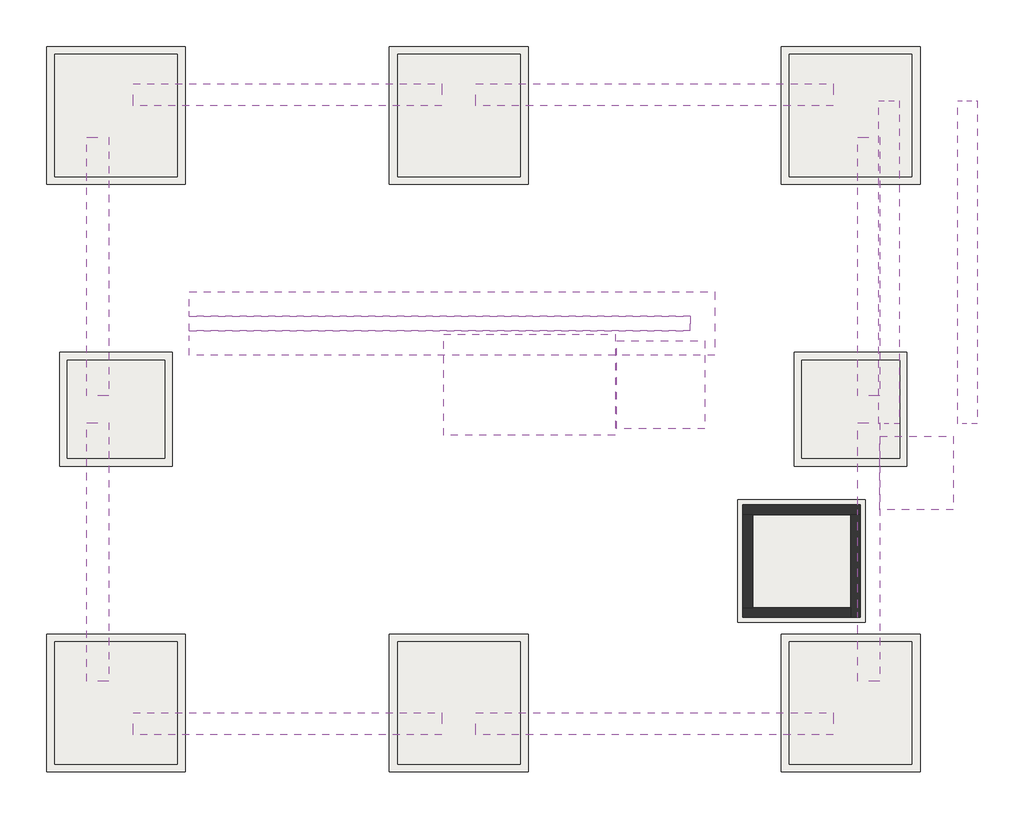
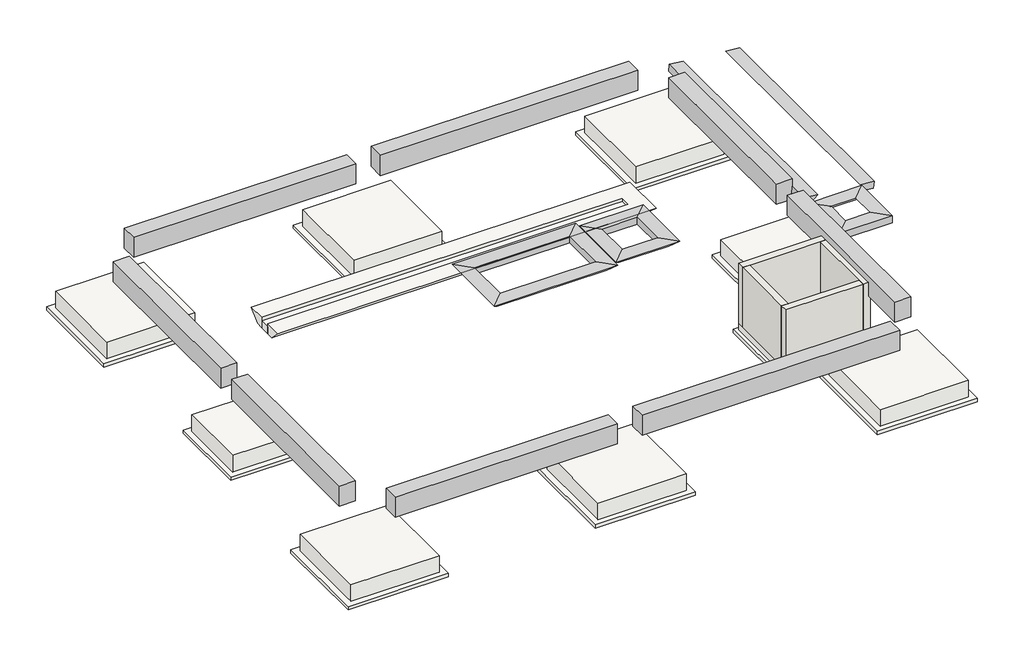
# One storey: 20 slabs, 7 beams, 5 proxies, 4 walls, 1 member.
# Revit data of these elements (continued)
# Type "FT112-Footing-Rectangular : FT112_2500x2500x500" (continued)
#   Foundation Thickness = 500 mm
#   hec_material3 [instance default] = none
#   hec_material2 [instance default] = A03AE056-00001_Bitumen/Bituminous/Asphalt Coating
#   hec_material1 [instance default] = A03AC035-00001_Form Work (3 times in use)_Flat
#   Structural Material [instance default] = A03AC032-00007_Structural Concrete_Type1_25MPa-30Mpa
#   Assembly Code = ""
# Type "MF111_THK.200"
#   Type Comments = ""
#   Layers, outside or top first: 200 mm "A03AC032-00007_Structural Concrete_Type1_25MPa-30Mpa" (function 1); 0 mm "A03AC035-00001_Form Work (3 times in use)_Flat" (function 100); 0 mm "A03AE056-00001_Bitumen/Bituminous/Asphalt Coating" (function 100)
# Type "WA111-UG RC Wall 200mm"
#   Type Comments = ""
#   Layers, outside or top first: 0 mm "A03AE056-00001_Bitumen/Bituminous/Asphalt Coating" (function 100); 200 mm "A03AC032-00007_Structural Concrete_Type1_25MPa-30Mpa" (function 1); 0 mm "A03AC035-00001_Form Work (3 times in use)_Flat" (function 100)
# Elements 1, 2, 3, 4, 5, 6, 7 (IfcBeam, "Concrete-Rectangular-Beam : BM112_450x600_UG")
#   Comments = ""
#   F01) Building Name = "Fire Water Pump Building"
#   F11) Project Building Tag_Type-1 = ""
#   F12) Project Building Tag_Type-2 = ""
#   F13) Project Facility Code = "621"
#   F21) Structural Type = "Steel"
#   F31) Standard Building Code = "E204"
#   F41) Discipline = "Architecture"
#   F51) Plan Start Date-Engineering = "2018-09-14"
#   F52) Plan Finish Date-Engineering = "2019-12-02"
#   F53) Duration = "444"
#   W11) Activity ID = "T3C621AR3610"
#   W12) Activity Name = "Fire Water Pump BLDG - Pedestal/Girder (U/G)"
#   W13) Plan Start Date = "2018-11-20"
#   W14) Plan Finish Date = "2019-02-02"
#   hec_material3 = none
#   hec_material2 = A03AE056-00001_Bitumen/Bituminous/Asphalt Coating
#   hec_material1 = A03AC035-00001_Form Work (3 times in use)_Flat
#   Structural Material = A03AC032-00007_Structural Concrete_Type1_25MPa-30Mpa
#   Phase Created = New Construction
#   Materials on its faces: "A03AC032-00007_Structural Concrete_Type1_25MPa-30Mpa"
# Elements 8, 9, 12 (IfcBuildingElementProxy, "Slab Edge")
#   Phase Created = New Construction
#   Materials on its faces: "Default Floor"
# Element 10 (IfcBuildingElementProxy, "Slab Edge")
#   built-in parameter 1001817 = -0.0996583 (stored number, unit not read)
#   Phase Created = New Construction
#   Materials on its faces: "Default Floor"
# Element 11 (IfcBuildingElementProxy, "Slab Edge")
#   built-in parameter 1001817 = 0.0996583 (stored number, unit not read)
#   Phase Created = New Construction
#   Materials on its faces: "Default Floor"
# Element 13 (IfcMember, "Concrete-Rectangular-Beam : BM112_450x600_UG")
#   Comments = ""
#   F01) Building Name = "Fire Water Pump Building"
#   F11) Project Building Tag_Type-1 = ""
#   F12) Project Building Tag_Type-2 = ""
#   F13) Project Facility Code = "621"
#   F21) Structural Type = "Steel"
#   F31) Standard Building Code = "E204"
#   F41) Discipline = "Architecture"
#   F51) Plan Start Date-Engineering = "2018-09-14"
#   F52) Plan Finish Date-Engineering = "2019-12-02"
#   F53) Duration = "444"
#   W11) Activity ID = "T3C621AR3610"
#   W12) Activity Name = "Fire Water Pump BLDG - Pedestal/Girder (U/G)"
#   W13) Plan Start Date = "2018-11-20"
#   W14) Plan Finish Date = "2019-02-02"
#   hec_material3 = none
#   hec_material2 = A03AE056-00001_Bitumen/Bituminous/Asphalt Coating
#   hec_material1 = A03AC035-00001_Form Work (3 times in use)_Flat
#   Structural Material = A03AC032-00007_Structural Concrete_Type1_25MPa-30Mpa
#   Phase Created = New Construction
#   Materials on its faces: "A03AC032-00007_Structural Concrete_Type1_25MPa-30Mpa"
# Elements 14, 15, 16, 17, 18, 19, 20, 21, 22 (IfcSlab, "SL101_Lean Floor_100")
#   Comments = ""
#   F01) Building Name = "Fire Water Pump Building"
#   F11) Project Building Tag_Type-1 = ""
#   F12) Project Building Tag_Type-2 = ""
#   F13) Project Facility Code = "621"
#   F21) Structural Type = "Steel"
#   F31) Standard Building Code = "E204"
#   F41) Discipline = "Architecture"
#   F51) Plan Start Date-Engineering = "2018-09-14"
#   F52) Plan Finish Date-Engineering = "2019-12-02"
#   F53) Duration = "444"
#   W11) Activity ID = "T3C621AR3110"
#   W12) Activity Name = "Fire Water Pump BLDG - Building Foundation"
#   W13) Plan Start Date = "2018-10-02"
#   W14) Plan Finish Date = "2018-11-24"
#   TMP_Element Name = "SS2"
#   Height Offset From Level = 0 mm
#   built-in parameter 1001954 = 1
#   Phase Created = New Construction
#   Materials on its faces: "A03AC034-00004_Lean Concrete (including Form work)"
# Element 23 (IfcSlab, "Ditch Wall 1 : Ditch Wall 1")
#   Phase Created = New Construction
#   Materials on its faces: "A03AC032-00007_Structural Concrete_Type1_25MPa-30Mpa"
# Element 24 (IfcSlab, "Ditch 2 : Ditch 2")
#   Phase Created = New Construction
#   Materials on its faces: "A03AC032-00007_Structural Concrete_Type1_25MPa-30Mpa"
# Elements 25, 26 (IfcSlab, "FT112-Footing-Rectangular : FT112_2000x2000x500")
#   Comments = ""
#   Mark = "F3"
#   F01) Building Name = "Fire Water Pump Building"
#   F11) Project Building Tag_Type-1 = ""
#   F12) Project Building Tag_Type-2 = ""
#   F13) Project Facility Code = "621"
#   F21) Structural Type = "Steel"
#   F31) Standard Building Code = "E204"
#   F41) Discipline = "Architecture"
#   F51) Plan Start Date-Engineering = "2018-09-14"
#   F52) Plan Finish Date-Engineering = "2019-12-02"
#   F53) Duration = "444"
#   W11) Activity ID = "T3C621AR3110"
#   W12) Activity Name = "Fire Water Pump BLDG - Building Foundation"
#   W13) Plan Start Date = "2018-10-02"
#   W14) Plan Finish Date = "2018-11-24"
#   Structural Material = 콘크리트 - 현장타설 콘크리트
#   Phase Created = New Construction
#   Materials on its faces: "콘크리트 - 현장타설 콘크리트"
# Elements 27, 28, 30, 31 (IfcSlab, "FT112-Footing-Rectangular : FT112_2500x2500x500")
#   Comments = ""
#   Mark = "F2"
#   F01) Building Name = "Fire Water Pump Building"
#   F11) Project Building Tag_Type-1 = ""
#   F12) Project Building Tag_Type-2 = ""
#   F13) Project Facility Code = "621"
#   F21) Structural Type = "Steel"
#   F31) Standard Building Code = "E204"
#   F41) Discipline = "Architecture"
#   F51) Plan Start Date-Engineering = "2018-09-14"
#   F52) Plan Finish Date-Engineering = "2019-12-02"
#   F53) Duration = "444"
#   W11) Activity ID = "T3C621AR3110"
#   W12) Activity Name = "Fire Water Pump BLDG - Building Foundation"
#   W13) Plan Start Date = "2018-10-02"
#   W14) Plan Finish Date = "2018-11-24"
#   Structural Material = 콘크리트 - 현장타설 콘크리트
#   Phase Created = New Construction
#   Materials on its faces: "콘크리트 - 현장타설 콘크리트"
# Elements 29, 32 (IfcSlab, "FT112-Footing-Rectangular : FT112_2500x2500x500")
#   Comments = ""
#   Mark = "F1"
#   F01) Building Name = "Fire Water Pump Building"
#   F11) Project Building Tag_Type-1 = ""
#   F12) Project Building Tag_Type-2 = ""
#   F13) Project Facility Code = "621"
#   F21) Structural Type = "Steel"
#   F31) Standard Building Code = "E204"
#   F41) Discipline = "Architecture"
#   F51) Plan Start Date-Engineering = "2018-09-14"
#   F52) Plan Finish Date-Engineering = "2019-12-02"
#   F53) Duration = "444"
#   W11) Activity ID = "T3C621AR3110"
#   W12) Activity Name = "Fire Water Pump BLDG - Building Foundation"
#   W13) Plan Start Date = "2018-10-02"
#   W14) Plan Finish Date = "2018-11-24"
#   Structural Material = 콘크리트 - 현장타설 콘크리트
#   Phase Created = New Construction
#   Materials on its faces: "콘크리트 - 현장타설 콘크리트"
# Element 33 (IfcSlab, "MF111_THK.200")
#   Comments = ""
#   F01) Building Name = "Fire Water Pump Building"
#   F11) Project Building Tag_Type-1 = ""
#   F12) Project Building Tag_Type-2 = ""
#   F13) Project Facility Code = "621"
#   F21) Structural Type = "Steel"
#   F31) Standard Building Code = "E204"
#   F41) Discipline = "Architecture"
#   F51) Plan Start Date-Engineering = "2018-09-14"
#   F52) Plan Finish Date-Engineering = "2019-12-02"
#   F53) Duration = "444"
#   W11) Activity ID = "T3C621AR3110"
#   W12) Activity Name = "Fire Water Pump BLDG - Building Foundation"
#   W13) Plan Start Date = "2018-10-02"
#   W14) Plan Finish Date = "2018-11-24"
#   Height Offset From Level = 200 mm
#   built-in parameter 1001954 = 1
#   Phase Created = New Construction
#   Materials on its faces: "A03AE056-00001_Bitumen/Bituminous/Asphalt Coating", "A03AC032-00007_Structural Concrete_Type1_25MPa-30Mpa"
# Elements 34, 35, 36 (IfcWall, "WA111-UG RC Wall 200mm")
#   Comments = ""
#   F01) Building Name = "Fire Water Pump Building"
#   F11) Project Building Tag_Type-1 = ""
#   F12) Project Building Tag_Type-2 = ""
#   F13) Project Facility Code = "621"
#   F21) Structural Type = "Steel"
#   F31) Standard Building Code = "E204"
#   F41) Discipline = "Architecture"
#   F51) Plan Start Date-Engineering = "2018-09-14"
#   F52) Plan Finish Date-Engineering = "2019-12-02"
#   F53) Duration = "444"
#   W11) Activity ID = "T3C621AR3610"
#   W12) Activity Name = "Fire Water Pump BLDG - Pedestal/Girder (U/G)"
#   W13) Plan Start Date = "2018-11-20"
#   W14) Plan Finish Date = "2019-02-02"
#   built-in parameter 1001111 = 200 mm
#   Top Offset = 0 mm
#   Base Offset = 200 mm
#   wall height = 1800 mm
#   Phase Created = New Construction
#   Base Constraint = 1.B.O.F (FL -2200)
#   Top Constraint = 2.G.L (FL -200)
#   Materials on its faces: "A03AC032-00007_Structural Concrete_Type1_25MPa-30Mpa", "Default Wall"
# Element 37 (IfcWall, "WA111-UG RC Wall 200mm")
#   Comments = ""
#   F01) Building Name = "Fire Water Pump Building"
#   F11) Project Building Tag_Type-1 = ""
#   F12) Project Building Tag_Type-2 = ""
#   F13) Project Facility Code = "621"
#   F21) Structural Type = "Steel"
#   F31) Standard Building Code = "E204"
#   F41) Discipline = "Architecture"
#   F51) Plan Start Date-Engineering = "2018-09-14"
#   F52) Plan Finish Date-Engineering = "2019-12-02"
#   F53) Duration = "444"
#   W11) Activity ID = "T3C621AR3610"
#   W12) Activity Name = "Fire Water Pump BLDG - Pedestal/Girder (U/G)"
#   W13) Plan Start Date = "2018-11-20"
#   W14) Plan Finish Date = "2019-02-02"
#   built-in parameter 1001111 = 200 mm
#   Top Offset = 0 mm
#   Base Offset = 200 mm
#   wall height = 1800 mm
#   Phase Created = New Construction
#   Base Constraint = 1.B.O.F (FL -2200)
#   Top Constraint = 2.G.L (FL -200)
#   Materials on its faces: "Default Wall", "A03AC032-00007_Structural Concrete_Type1_25MPa-30Mpa"
# Materials
#   "콘크리트 - 현장타설 콘크리트": class "콘크리트", colour RGB 192 192 192, transparency 0, Cost = 0
#   "A03AC034-00004_Lean Concrete (including Form work)": class "Concrete", colour RGB 176 176 176, transparency 0, Description = "Plain Conc.", W00) Work Master Code = "A03AC034-00004", W01) Work Master_Lv1 = "Concrete Work", W02) Work Master_Lv2 = "Substructure Work", W03) Work Master_Spec.1 = "Lean Concrete (including Form work)", W04) Work Master_Spec.2 = "Cement Type-1", W05) Work Master_Spec.3 = "10MPa < F'c (Cylinder Strength) ≤ 20MPa", Cost = 0
#   "A03AE056-00001_Bitumen/Bituminous/Asphalt Coating": class "Generic", colour RGB 17 17 17, transparency 0, Description = "Damp-proofing", W00) Work Master Code = "A03AE056-00001", W01) Work Master_Lv1 = "Concrete Work", W02) Work Master_Lv2 = "Concrete Protective Coating (U/G)", W03) Work Master_Spec.1 = "Bitumen/Bituminous/Asphalt Coating", Cost = 0
#   "A03AC035-00001_Form Work (3 times in use)_Flat": class "Wood", colour RGB 149 120 74, transparency 0, Description = "Plywood", W00) Work Master Code = "A03AC035-00001", W01) Work Master_Lv1 = "Concrete Work", W02) Work Master_Lv2 = "Substructure Work", W03) Work Master_Spec.1 = "Form Work (3 times in use)", W04) Work Master_Spec.2 = "Flat Form", W05) Work Master_Spec.3 = "Dressed Lumber, Plywood or Steel Form(Wood Planks are not Allowed) incl. Chamfer", Cost = 0
#   "A03AC032-00007_Structural Concrete_Type1_25MPa-30Mpa": class "Concrete", colour RGB 176 176 176, transparency 0, Keynote = "09910.A1", Description = "Reinf. Conc.", W00) Work Master Code = "A03AC032-00007", W01) Work Master_Lv1 = "Concrete Work", W02) Work Master_Lv2 = "Substructure Work", W03) Work Master_Spec.1 = "Structural Concrete", W04) Work Master_Spec.2 = "Cement Type-1", W05) Work Master_Spec.3 = "25MPa < F'c (Cylinder Strength) ≤ 30MPa", Cost = 0
#   "Default Floor": class "Miscellaneous", colour RGB 80 80 80, transparency 0
#   "Default Wall": class "Miscellaneous", colour RGB 80 80 80, transparency 0
